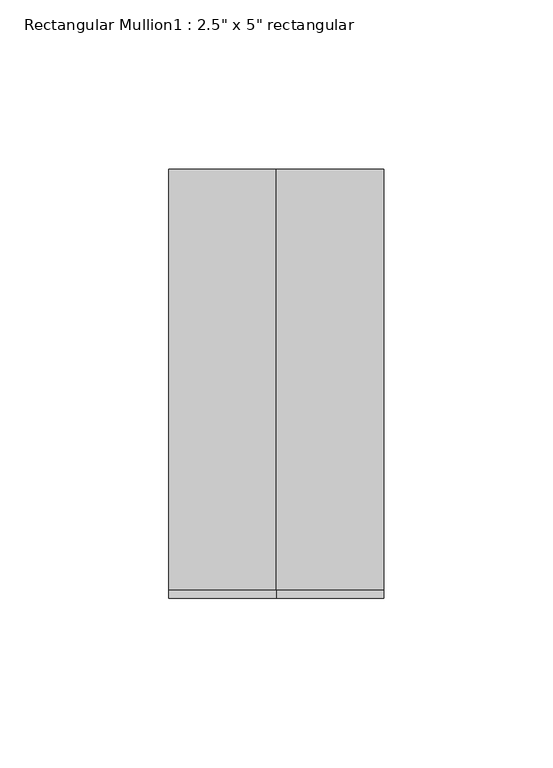
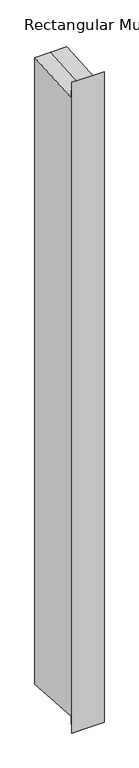
"""IFC4 building model written with IfcOpenShell, lengths in millimetres: member geometry."""

from ifc_helpers import new_model, si_unit, origin, place, context, project, spatial, faceted_brep, source, transform, mapped, element, save


def member_d66ac510(model_context):
    return source(origin(), model_context, "Body", "Brep", [
        faceted_brep([(-31.75, 63.5, 4.4114583), (0.0, 63.5, 4.4114583), (31.75, 63.5, 4.4114583), (31.75, 63.5, -1307.1798222), (0.0, 63.5, -1307.1798222), (-31.75, 63.5, -1307.1798222), (-31.75, -63.5, 29.5074223), (-31.75, -61.1020145, -4.4004678), (-31.75, -61.1020145, -1298.3678961), (-31.75, -63.5, -1332.2757861), (31.75, -63.5, 29.5074223), (0.0, -63.5, 29.5074223), (0.0, -63.5, -1332.2757861), (31.75, -63.5, -1332.2757861), (31.75, -61.1020145, -4.4004678), (31.75, -61.1020145, -1298.3678961), (0.0, -61.1020145, -4.4004678), (0.0, -61.1020145, -1298.3678961)], [[[0, 1, 2, 3, 4, 5]], [[6, 7, 0, 5, 8, 9]], [[10, 11, 6, 9, 12, 13]], [[2, 14, 10, 13, 15, 3]], [[2, 1, 16, 14]], [[1, 0, 7, 16]], [[7, 6, 11, 16]], [[11, 10, 14, 16]], [[3, 15, 17, 4]], [[15, 13, 12, 17]], [[12, 9, 8, 17]], [[8, 5, 4, 17]]]),
    ])


if __name__ == "__main__":
    model = new_model("IFC4")
    model_context = context("Model", 3, world=origin())
    ifc_project = project(units=[si_unit("LENGTHUNIT", "METRE", prefix="MILLI")], contexts=[model_context])
    site = spatial("IfcSite", under=ifc_project)
    building = spatial("IfcBuilding", under=site)
    placement = place(None, origin())
    member_shape = member_d66ac510(model_context)
    element("IfcMember", 1, ObjectType="Rectangular Mullion1 : 2.5\" x 5\" rectangular", at=placement, inside=building, context=model_context, shape_type="MappedRepresentation", body=[
        mapped(member_shape, transform((0.0, 0.0, 0.0), x_axis=(1.0, 0.0, 0.0), y_axis=(0.0, 1.0, 0.0), z_axis=(0.0, 0.0, 1.0))),
    ])
    save(model, "model.ifc")

# Revit data of these elements
# Type "Rectangular Mullion1 : 2.5\" x 5\" rectangular"
#   built-in parameter 1007304 = 0.416667 (stored number, unit not read)
#   built-in parameter 1007301 = 0.104167 (stored number, unit not read)
#   built-in parameter 1007300 = 0.104167 (stored number, unit not read)
# Element 1 (IfcMember, "Rectangular Mullion1 : 2.5\" x 5\" rectangular")
#   Materials on its faces: "support-frame"
# Materials
#   "support-frame": class "Unassigned", colour RGB 233 233 233, transparency 0, Cost = 0
